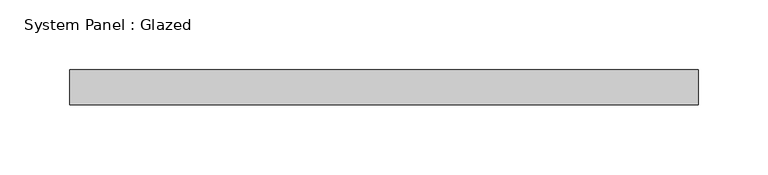
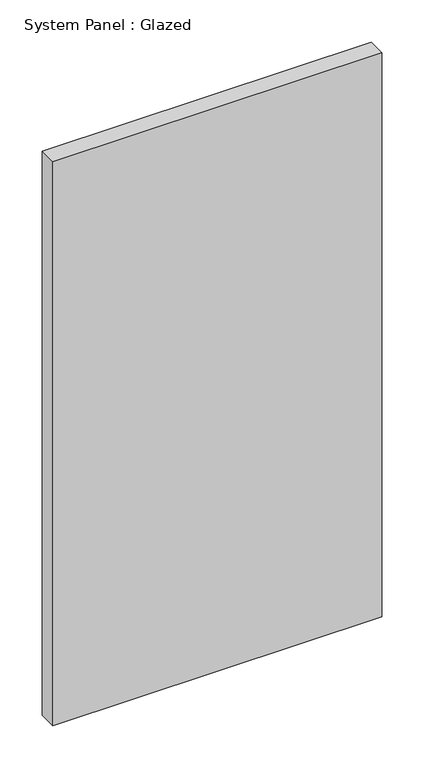
"""IFC4 building model written with IfcOpenShell, lengths in millimetres: plate geometry, System Panel : Glazed."""

from ifc_helpers import new_model, si_unit, origin, origin_with_axes, place, context, project, spatial, polyline, outline, extrude, source, transform, mapped, element, save


def system_panel_glazed_b5f8ad4b(model_context):
    return source(origin(), model_context, "Body", "SweptSolid", [
        extrude(outline(polyline([(225.9820235, 19.05), (-225.9820235, 19.05), (-225.9820235, 44.45), (225.9820235, 44.45), (225.9820235, 19.05)])), origin_with_axes(), (0.0, 0.0, 1.0), 819.15),
    ])


if __name__ == "__main__":
    model = new_model("IFC4")
    model_context = context("Model", 3, world=origin())
    ifc_project = project(units=[si_unit("LENGTHUNIT", "METRE", prefix="MILLI")], contexts=[model_context])
    site = spatial("IfcSite", under=ifc_project)
    building = spatial("IfcBuilding", under=site)
    placement = place(None, origin())
    system_panel_glazed_shape = system_panel_glazed_b5f8ad4b(model_context)
    element("IfcPlate", 1, ObjectType="System Panel : Glazed", at=placement, inside=building, context=model_context, shape_type="MappedRepresentation", body=[
        mapped(system_panel_glazed_shape, transform((0.0, 0.0, 0.0), x_axis=(1.0, 0.0, 0.0), y_axis=(0.0, 1.0, 0.0), z_axis=(0.0, 0.0, 1.0))),
    ])
    save(model, "model.ifc")

# Revit data of these elements
# Element 1 (IfcPlate, "System Panel : Glazed")
#   Materials on its faces: "Glass"
# Materials
#   "Glass": class "Glass", colour RGB 0 128 192, transparency 0.75
